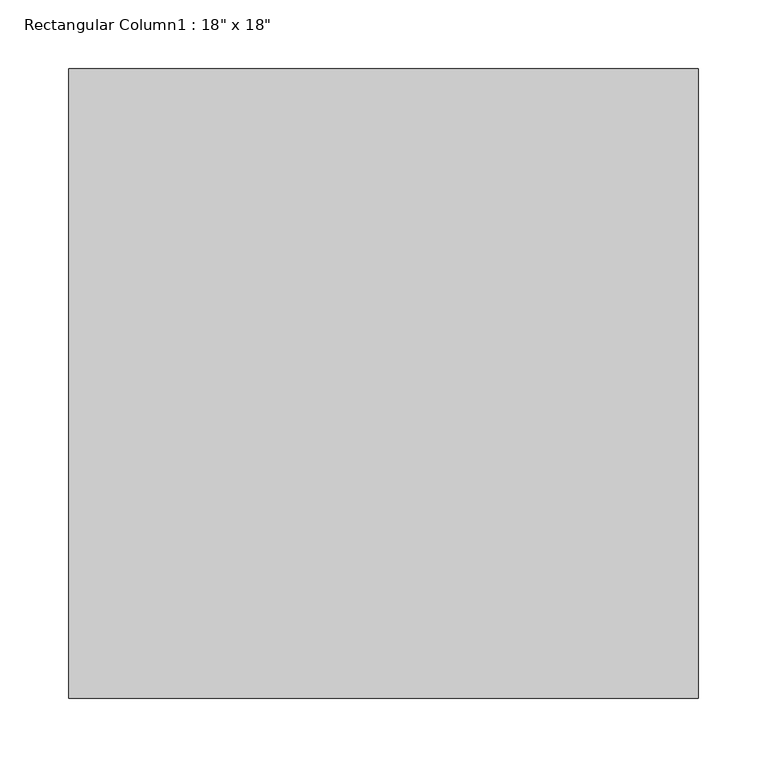
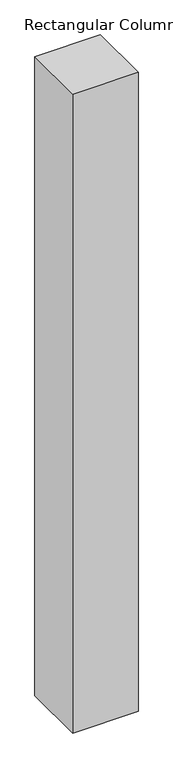
"""IFC4 building model written with IfcOpenShell, lengths in millimetres: column geometry."""

from ifc_helpers import new_model, si_unit, frame, origin, place, context, project, spatial, polyline, outline, extrude, source, transform, mapped, element, save


def column_f6efb254(model_context):
    return source(origin(), model_context, "Body", "SweptSolid", [
        extrude(outline(polyline([(228.6, 228.6), (228.6, -228.6), (-228.6, -228.6), (-228.6, 228.6), (228.6, 228.6)])), frame((0.0, 0.0, 5486.4), z_axis=(0.0, 0.0, 1.0), x_axis=(1.0, 0.0, 0.0)), (0.0, 0.0, 1.0), 4724.4),
    ])


if __name__ == "__main__":
    model = new_model("IFC4")
    model_context = context("Model", 3, world=origin())
    ifc_project = project(units=[si_unit("LENGTHUNIT", "METRE", prefix="MILLI")], contexts=[model_context])
    site = spatial("IfcSite", under=ifc_project)
    building = spatial("IfcBuilding", under=site)
    placement = place(None, origin())
    column_shape = column_f6efb254(model_context)
    element("IfcColumn", 1, ObjectType="Rectangular Column1 : 18\" x 18\"", at=placement, inside=building, context=model_context, shape_type="MappedRepresentation", body=[
        mapped(column_shape, transform((0.0, 0.0, 0.0), x_axis=(1.0, 0.0, 0.0), y_axis=(0.0, 1.0, 0.0), z_axis=(0.0, 0.0, 1.0))),
    ])
    save(model, "model.ifc")

# Revit data of these elements
# Type "Rectangular Column1 : 18\" x 18\""
#   Depth = 1' - 6"
#   Width = 1' - 6"
